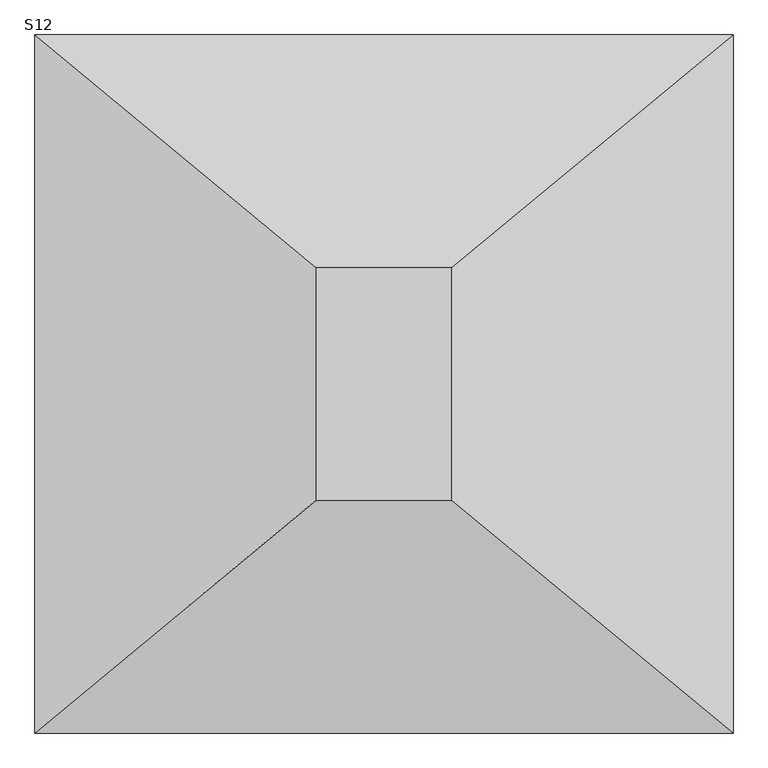
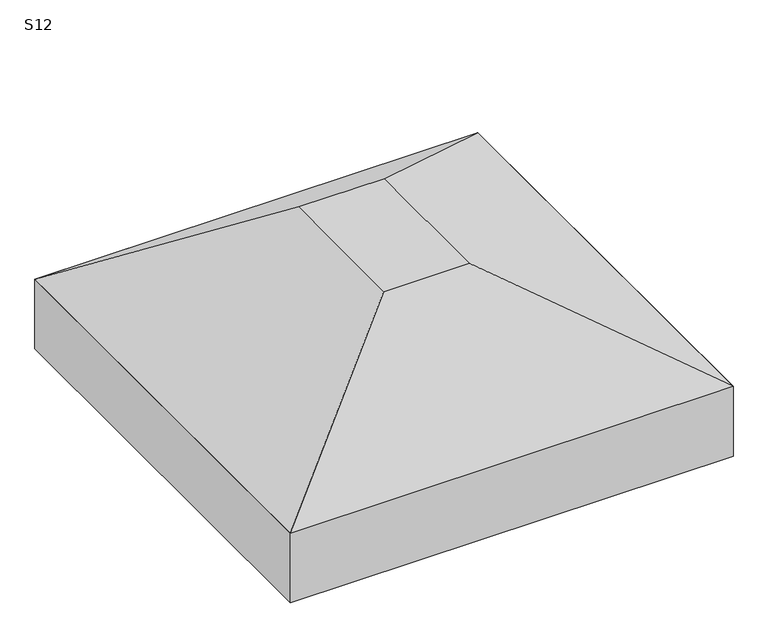
"""IFC4 building model written with IfcOpenShell, lengths in millimetres: fastener geometry, TQS - Sapata : S12."""

from ifc_helpers import new_model, si_unit, frame, origin, place, context, project, spatial, polyline, outline, extrude, faceted_brep, source, transform, mapped, element, save


def s12_1e6d1b45(model_context):
    return source(origin(), model_context, "Body", "SolidModel", [
        faceted_brep([(-55.0, 50.0, 0.0), (-345.0, 50.0, 0.0), (-345.0, -450.0, 0.0), (-55.0, -450.0, 0.0), (550.0, 550.0, -350.0), (550.0, -950.0, -350.0), (-950.0, -950.0, -350.0), (-950.0, 550.0, -350.0)], [[[0, 1, 2, 3]], [[4, 5, 6, 7]], [[4, 7, 1, 0]], [[7, 6, 2, 1]], [[6, 5, 3, 2]], [[5, 4, 0, 3]]]),
        extrude(outline(polyline([(550.0, 550.0), (550.0, -950.0), (-950.0, -950.0), (-950.0, 550.0), (550.0, 550.0)])), frame((0.0, 0.0, -600.0), z_axis=(0.0, 0.0, 1.0), x_axis=(1.0, 0.0, 0.0)), (0.0, 0.0, 1.0), 250.0),
    ])


if __name__ == "__main__":
    model = new_model("IFC4")
    model_context = context("Model", 3, world=origin())
    ifc_project = project(units=[si_unit("LENGTHUNIT", "METRE", prefix="MILLI")], contexts=[model_context])
    site = spatial("IfcSite", under=ifc_project)
    building = spatial("IfcBuilding", under=site)
    placement = place(None, origin())
    s12_shape = s12_1e6d1b45(model_context)
    element("IfcFastener", 1, ObjectType="TQS - Sapata : S12", at=placement, inside=building, context=model_context, shape_type="MappedRepresentation", body=[
        mapped(s12_shape, transform((0.0, 0.0, 0.0), x_axis=(1.0, 0.0, 0.0), y_axis=(0.0, 1.0, 0.0), z_axis=(0.0, 0.0, 1.0))),
    ])
    save(model, "model.ifc")

# Revit data of these elements
# Type "TQS - Sapata : S12"
#   TY = 0.50 m
#   TX = 0.29 m
#   HS = 0.60 m
#   H0 = 0.25 m
#   EXCYABS = 0.75 m
#   EXCY = 0.00 m
#   EXCXABS = 0.75 m
#   EXCX = 0.00 m
#   DIMY = 1.50 m
#   DIMX = 1.50 m
#   Material estrutural = Concreto - Concreto concretado no local
#   Width = 0
#   Length = 0
# Element 1 (IfcFastener, "TQS - Sapata : S12")
#   Materials on its faces: "Concreto - Concreto concretado no local"
# Materials
#   "Concreto - Concreto concretado no local": class "Concreto", colour RGB 192 192 192, transparency 0
